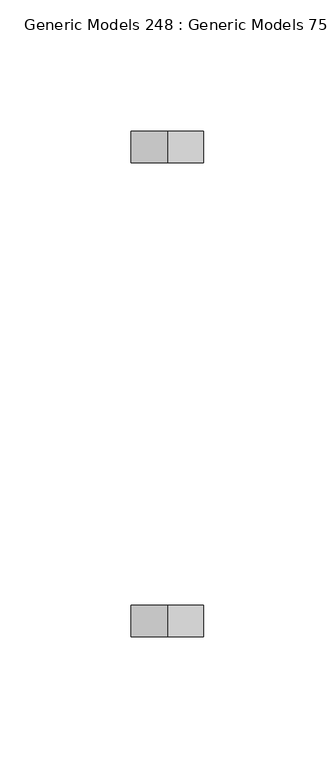
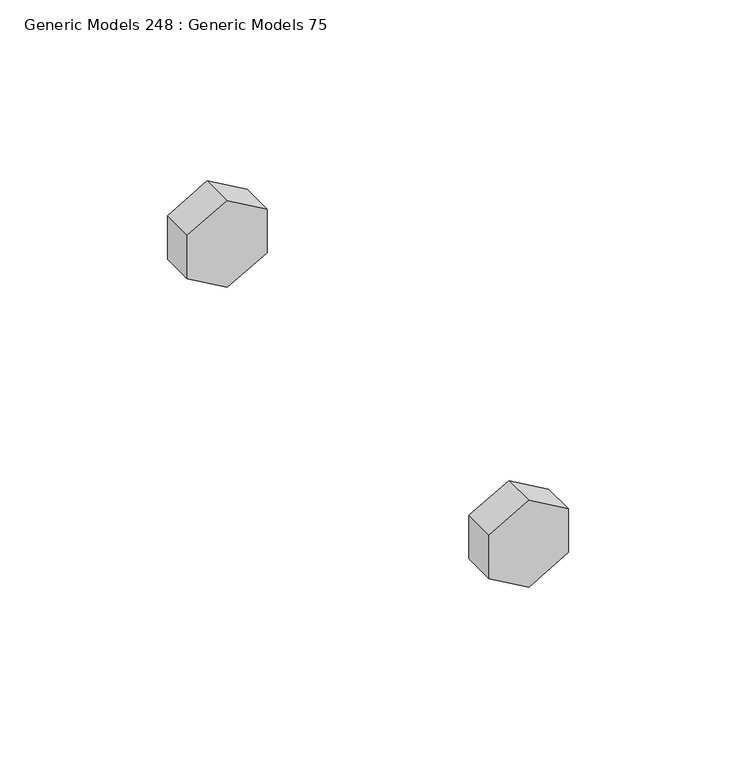
"""IFC4 building model written with IfcOpenShell, lengths in millimetres: proxy geometry, Generic Models 248 : Generic Models 75."""

from ifc_helpers import new_model, si_unit, frame, origin, place, context, project, spatial, polyline, outline, extrude, source, transform, mapped, element, save


def generic_models_248_generic_models_75_7ee3556c(model_context):
    return source(origin(), model_context, "Body", "SweptSolid", [
        extrude(outline(polyline([(269222.3462802, 31975.9942029), (269206.5097067, 31975.9942029), (269198.59142, 31989.7090778), (269206.5097067, 32003.4239528), (269222.3462802, 32003.4239528), (269230.264567, 31989.7090778), (269222.3462802, 31975.9942029)])), frame((0.0, 30858.4781612, 0.0), z_axis=(0.0, 1.0, 0.0), x_axis=(0.0, 0.0, 1.0)), (0.0, 0.0, 1.0), 11.90625),
        extrude(outline(polyline([(269222.3462802, 31975.9942029), (269206.5097067, 31975.9942029), (269198.59142, 31989.7090778), (269206.5097067, 32003.4239528), (269222.3462802, 32003.4239528), (269230.264567, 31989.7090778), (269222.3462802, 31975.9942029)])), frame((0.0, 30678.2969112, 0.0), z_axis=(0.0, 1.0, 0.0), x_axis=(0.0, 0.0, 1.0)), (0.0, 0.0, 1.0), 11.90625),
    ])


if __name__ == "__main__":
    model = new_model("IFC4")
    model_context = context("Model", 3, world=origin())
    ifc_project = project(units=[si_unit("LENGTHUNIT", "METRE", prefix="MILLI")], contexts=[model_context])
    site = spatial("IfcSite", under=ifc_project)
    building = spatial("IfcBuilding", under=site)
    placement = place(None, origin())
    generic_models_248_generic_models_75_shape = generic_models_248_generic_models_75_7ee3556c(model_context)
    element("IfcBuildingElementProxy", 1, Name="Generic Models 248 : Generic Models 75", ObjectType="Generic Models 248 : Generic Models 75", at=placement, inside=building, context=model_context, shape_type="MappedRepresentation", body=[
        mapped(generic_models_248_generic_models_75_shape, transform((0.0, 0.0, 0.0), x_axis=(1.0, 0.0, 0.0), y_axis=(0.0, 1.0, 0.0), z_axis=(0.0, 0.0, 1.0))),
    ])
    save(model, "model.ifc")

# Revit data of these elements
# Element 1 (IfcBuildingElementProxy, "Generic Models 248 : Generic Models 75")
#   Materials on its faces: "3/4\" GALV. THRU BOLTS"
# Materials
#   "3/4\" GALV. THRU BOLTS": class "Generic", colour RGB 105 69 171, transparency 0, Cost = 0
